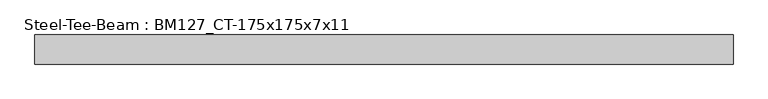
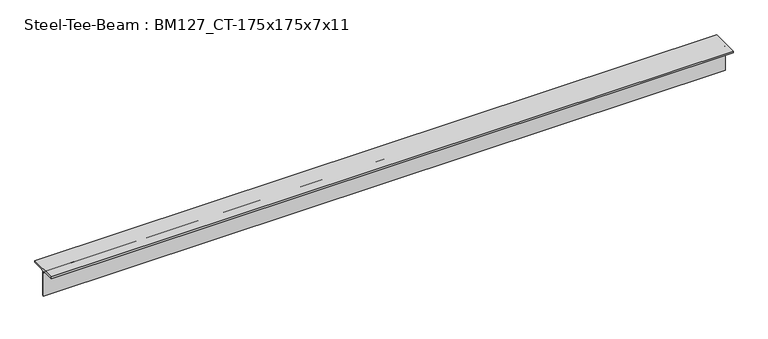
"""IFC4 building model written with IfcOpenShell, lengths in millimetres: beam geometry, Steel-Tee-Beam : BM127_CT-175x175x7x11."""

from ifc_helpers import new_model, si_unit, point, frame, frame_2d, origin, place, context, project, spatial, polyline, circle_curve, trimmed, segment, composite_curve, outline, extrude, source, transform, mapped, element, save


def steel_tee_beam_bm127_ct_175x175x7x11_36c48f08(model_context):
    return source(origin(), model_context, "Body", "SweptSolid", [
        extrude(outline(composite_curve([segment(polyline([(87.5, 87.5), (87.5, 76.5), (17.5, 76.5)]), True, "CONTINUOUS"), segment(trimmed(circle_curve(frame_2d((17.5, 62.5)), 14.0), [point((17.5, 76.5))], [point((3.5, 62.5))], True, "CARTESIAN"), True, "CONTINUOUS"), segment(polyline([(3.5, 62.5), (3.5, -87.5), (-3.5, -87.5), (-3.5, 62.5)]), True, "CONTINUOUS"), segment(trimmed(circle_curve(frame_2d((-17.5, 62.5)), 14.0), [point((-3.5, 62.5))], [point((-17.5, 76.5))], True, "CARTESIAN"), True, "CONTINUOUS"), segment(polyline([(-17.5, 76.5), (-87.5, 76.5), (-87.5, 87.5), (87.5, 87.5)]), True, "CONTINUOUS")], self_intersect=False)), frame((-1998.4928423, 0.0, 0.0), z_axis=(1.0, 0.0, 0.0), x_axis=(0.0, 1.0, 0.0)), (0.0, 0.0, 1.0), 4194.118334),
    ])


if __name__ == "__main__":
    model = new_model("IFC4")
    model_context = context("Model", 3, world=origin())
    ifc_project = project(units=[si_unit("LENGTHUNIT", "METRE", prefix="MILLI")], contexts=[model_context])
    site = spatial("IfcSite", under=ifc_project)
    building = spatial("IfcBuilding", under=site)
    placement = place(None, origin())
    steel_tee_beam_bm127_ct_175x175x7x11_shape = steel_tee_beam_bm127_ct_175x175x7x11_36c48f08(model_context)
    element("IfcBeam", 1, ObjectType="Steel-Tee-Beam : BM127_CT-175x175x7x11", at=placement, inside=building, context=model_context, shape_type="MappedRepresentation", body=[
        mapped(steel_tee_beam_bm127_ct_175x175x7x11_shape, transform((0.0, 0.0, 0.0), x_axis=(1.0, 0.0, 0.0), y_axis=(0.0, 1.0, 0.0), z_axis=(0.0, 0.0, 1.0))),
    ])
    save(model, "model.ifc")

# Revit data of these elements
# Type "Steel-Tee-Beam : BM127_CT-175x175x7x11"
#   Surface Area = 0.00 m²/m
#   Section Area = 31.57 cm²
#   Mass per Unit Length = 24.80 kg/m
#   Length [instance default] = 1524 mm
#   bf = 175 mm
#   d = 175 mm
#   k = 25 mm
#   kr = 14 mm
#   tf = 11 mm
#   tw = 7 mm
#   hec_material4 [instance default] = none
#   hec_material3 [instance default] = none
#   hec_material2 [instance default] = none
#   hec_material1 [instance default] = none
#   Structural Material [instance default] = Steel, 45-345
#   Assembly Code = ""
# Element 1 (IfcBeam, "Steel-Tee-Beam : BM127_CT-175x175x7x11")
#   hec_material3 = F01AC000-00002_Building/Shelter Fire Proofing Work_Intumescent Coating Type_1 hr. rating (UL 1709))
#   hec_material2 = S01AA010-00002_Main Steel Structure Fabrication Work_Shelter/Building_Steel Painting/Coating_for Fireproofed Steel Surface, Surface Preparation & Primer Coat
#   hec_material1 = S03AA029-00001_Main Steel Structure Erection Work_Shelter/Building_Light Steel
#   Structural Material = S01AA003-00001_Main Steel Structure Fabrication Work_Shelter/Building_Light Steel - Standard
#   Materials on its faces: "S01AA003-00001_Main Steel Structure Fabrication Work_Shelter/Building_Light Steel - Standard"
# Materials
#   "Steel, 45-345": class "Metal", colour RGB 189 187 185, transparency 0, Description = "Steel 345 MPa", Cost = 0
#   "S01AA003-00001_Main Steel Structure Fabrication Work_Shelter/Building_Light Steel - Standard": class "Metal", colour RGB 120 120 120, transparency 0, Comments = "(30KG/M>Weight)", Description = "Structural steel 50ksi", W00) Work Master Code = "S01AA003-00001", W01) Work Master_Lv1 = "Main Steel Structure Fabrication Work", W02) Work Master_Lv2 = "Shelter/Building", W03) Work Master_Spec.1 = "Light Steel - Standard (30KG/M>Weight)", Cost = 0
#   "F01AC000-00002_Building/Shelter Fire Proofing Work_Intumescent Coating Type_1 hr. rating (UL 1709))": class "Metal", colour RGB 255 128 128, transparency 0, Description = "Paint finished steel", W00) Work Master Code = "F01AC000-00002", W01) Work Master_Lv1 = "Building/Shelter Fire Proofing Work", W02) Work Master_Lv2 = "Intumescent Coating Type", W03) Work Master_Spec.1 = "1 hr. rating (UL 1709)", Cost = 0
#   "S01AA010-00002_Main Steel Structure Fabrication Work_Shelter/Building_Steel Painting/Coating_for Fireproofed Steel Surface, Surface Preparation & Primer Coat": class "Metal", colour RGB 120 120 120, transparency 0, Description = "Paint finished steel", W00) Work Master Code = "SS01AA010-00002", W01) Work Master_Lv1 = "Main Steel Structure Fabrication Work", W02) Work Master_Lv2 = "Shelter/Building", W03) Work Master_Spec.1 = "Steel Painting/Coating", W04) Work Master_Spec.2 = "for Fireproofed Steel Surface, Surface Preparation & Primer Coat", Cost = 0
#   "S03AA029-00001_Main Steel Structure Erection Work_Shelter/Building_Light Steel": class "Metal", colour RGB 120 120 120, transparency 0, Comments = "(30KG/M>Weight)", Description = "Structural steel 50ksi", W00) Work Master Code = "S03AA029-00001", W01) Work Master_Lv1 = "Main Steel Structure Erection Work", W02) Work Master_Lv2 = "Shelter/Building", W03) Work Master_Spec.1 = "Light Steel (30KG/M>Weight)", Cost = 0
